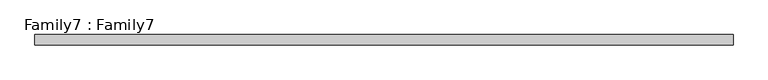
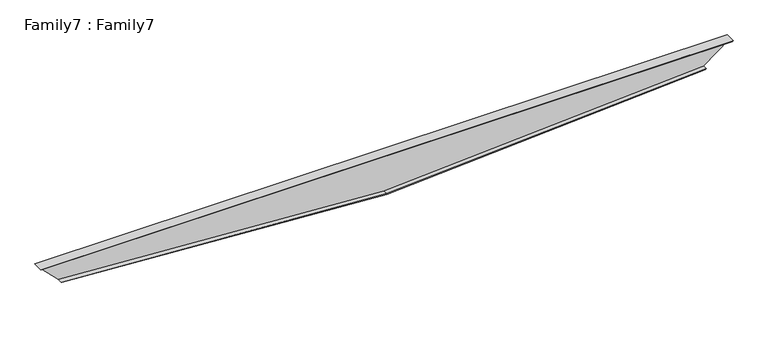
"""IFC4 building model written with IfcOpenShell, lengths in millimetres: beam geometry, Family7 : Family7."""

from ifc_helpers import new_model, si_unit, frame, origin, place, context, project, spatial, polyline, outline, extrude, source, transform, mapped, element, save


def family7_family7_c56ba9d3(model_context):
    return source(origin(), model_context, "Body", "SweptSolid", [
        extrude(outline(polyline([(-914.4, -14634.0702512), (-1828.8, 0.0), (-914.4, 14362.0989586), (-31.75, 15533.4150704), (-31.75, -15516.7202512), (-914.4, -14634.0702512)])), frame((0.0, -15.875, 0.0), z_axis=(0.0, 1.0, 0.0), x_axis=(0.0, 0.0, 1.0)), (0.0, 0.0, 1.0), 31.75),
        extrude(outline(polyline([(-914.4, 14362.0989586), (-1828.8, 0.0), (-914.4, -14634.0702512), (-948.3321476, -14600.1381036), (-1860.6130916, 0.0187468), (-949.1503311, 14315.9837117), (-914.4, 14362.0989586)])), frame((0.0, -228.6, 0.0), z_axis=(0.0, 1.0, 0.0), x_axis=(0.0, 0.0, 1.0)), (0.0, 0.0, 1.0), 457.2),
        extrude(outline(polyline([(-31.75, 15533.4150704), (0.0, 15575.5487435), (0.0, -15548.4702512), (-31.75, -15516.7202512), (-31.75, 15533.4150704)])), frame((0.0, -228.6, 0.0), z_axis=(0.0, 1.0, 0.0), x_axis=(0.0, 0.0, 1.0)), (0.0, 0.0, 1.0), 457.2),
    ])


if __name__ == "__main__":
    model = new_model("IFC4")
    model_context = context("Model", 3, world=origin())
    ifc_project = project(units=[si_unit("LENGTHUNIT", "METRE", prefix="MILLI")], contexts=[model_context])
    site = spatial("IfcSite", under=ifc_project)
    building = spatial("IfcBuilding", under=site)
    placement = place(None, origin())
    family7_family7_shape = family7_family7_c56ba9d3(model_context)
    element("IfcBeam", 1, ObjectType="Family7 : Family7", at=placement, inside=building, context=model_context, shape_type="MappedRepresentation", body=[
        mapped(family7_family7_shape, transform((0.0, 0.0, 0.0), x_axis=(1.0, 0.0, 0.0), y_axis=(0.0, 1.0, 0.0), z_axis=(0.0, 0.0, 1.0))),
    ])
    save(model, "model.ifc")

# Revit data of these elements
# Type "Family7 : Family7"
#   Width = 1' - 6"
#   Web_Thickness = 0' - 1 1/4"
#   Length [instance default] = 69' - 10"
#   Depth_Mid [instance default] = 6' - 0"
#   Depth_End = 3' - 0"
#   Angle_Right = 53.00°
#   Angle_Left = 45.00°
#   Structural Material [instance default] = none
# Element 1 (IfcBeam, "Family7 : Family7")
#   Structural Material = Steel
#   Materials on its faces: "Steel"
# Materials
#   "Steel": class "Metal", colour RGB 118 118 114, transparency 0, Description = "Steel, mill finish", Cost = 0
